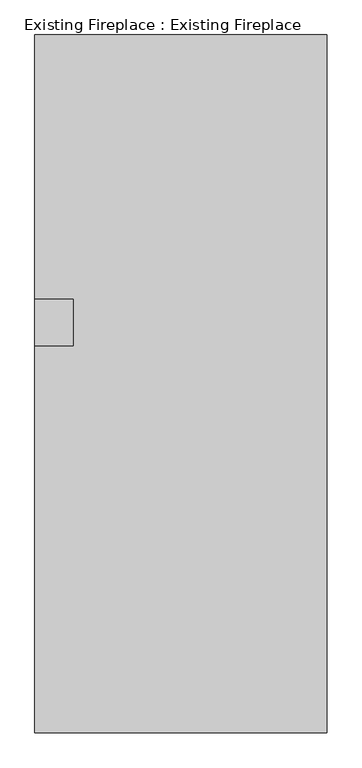
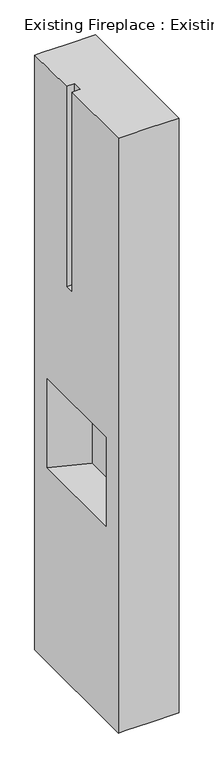
"""IFC4 building model written with IfcOpenShell, lengths in millimetres: proxy geometry, Existing Fireplace : Existing Fireplace."""

from ifc_helpers import new_model, si_unit, origin, place, context, project, spatial, faceted_brep, source, transform, mapped, element, save


def existing_fireplace_existing_fireplace_063a625f(model_context):
    return source(origin(), model_context, "Body", "Brep", [
        faceted_brep([(4450.2196932, 434.2888758, 5486.4), (4069.2196932, 434.2888758, 5486.4), (3764.4196932, 434.2888758, 5486.4), (3662.8196932, 434.2888758, 5486.4), (3662.8196932, -276.9111242, 5486.4), (3767.2567114, -276.9111242, 5486.4), (3767.2567114, -403.9111242, 5486.4), (3662.8196932, -403.9111242, 5486.4), (3662.8196932, -1445.3111242, 5486.4), (3764.4196932, -1445.3111242, 5486.4), (4069.2196932, -1445.3111242, 5486.4), (4450.2196932, -1445.3111242, 5486.4), (4450.2196932, 434.2888758, -2667.0), (4450.2196932, -1445.3111242, -2667.0), (4069.2196932, -1445.3111242, -2667.0), (3764.4196932, -1445.3111242, -2667.0), (3662.8196932, -1445.3111242, -2667.0), (3662.8196932, 434.2888758, -2667.0), (3764.4196932, 434.2888758, -2667.0), (4069.2196932, 434.2888758, -2667.0), (3662.8196932, -403.9111242, 2743.2), (3662.8196932, -276.9111242, 2743.2), (3662.8196932, 154.8888758, 0.0), (3662.8196932, 154.8888758, 1219.2), (3662.8196932, -1165.9111242, 1219.2), (3662.8196932, -1165.9111242, 0.0), (4145.4196932, -20.7631592, 1219.2), (4145.4196932, -990.2590891, 1219.2), (4145.4196932, -990.2590891, 0.0), (4145.4196932, -20.7631592, 0.0), (3767.2567114, -403.9111242, 2743.2), (3767.2567114, -276.9111242, 2743.2)], [[[0, 1, 2, 3, 4, 5, 6, 7, 8, 9, 10, 11]], [[12, 13, 14, 15, 16, 17, 18, 19]], [[3, 2, 1, 0, 12, 19, 18, 17]], [[3, 17, 16, 8, 7, 20, 21, 4], [22, 23, 24, 25]], [[11, 10, 9, 8, 16, 15, 14, 13]], [[0, 11, 13, 12]], [[24, 23, 26, 27]], [[25, 24, 27, 28]], [[27, 26, 29, 28]], [[23, 22, 29, 26]], [[22, 25, 28, 29]], [[6, 30, 20, 7]], [[31, 5, 4, 21]], [[30, 31, 21, 20]], [[30, 6, 5, 31]]]),
    ])


if __name__ == "__main__":
    model = new_model("IFC4")
    model_context = context("Model", 3, world=origin())
    ifc_project = project(units=[si_unit("LENGTHUNIT", "METRE", prefix="MILLI")], contexts=[model_context])
    site = spatial("IfcSite", under=ifc_project)
    building = spatial("IfcBuilding", under=site)
    placement = place(None, origin())
    existing_fireplace_existing_fireplace_shape = existing_fireplace_existing_fireplace_063a625f(model_context)
    element("IfcBuildingElementProxy", 1, Name="Existing Fireplace : Existing Fireplace", ObjectType="Existing Fireplace : Existing Fireplace", at=placement, inside=building, context=model_context, shape_type="MappedRepresentation", body=[
        mapped(existing_fireplace_existing_fireplace_shape, transform((0.0, 0.0, 0.0), x_axis=(1.0, 0.0, 0.0), y_axis=(0.0, 1.0, 0.0), z_axis=(0.0, 0.0, 1.0))),
    ])
    save(model, "model.ifc")
